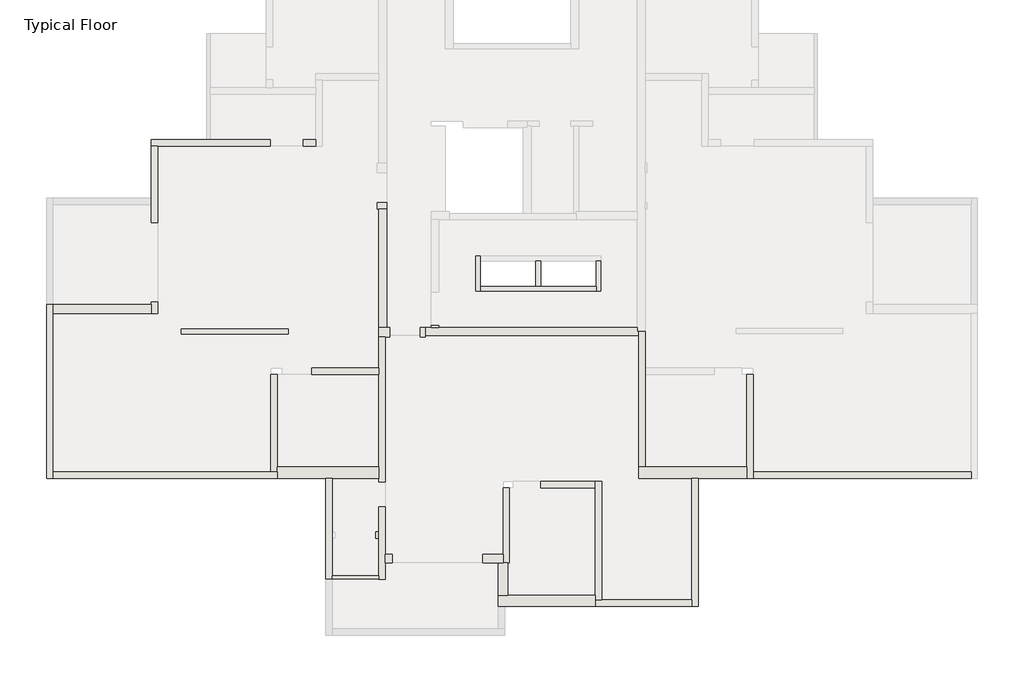
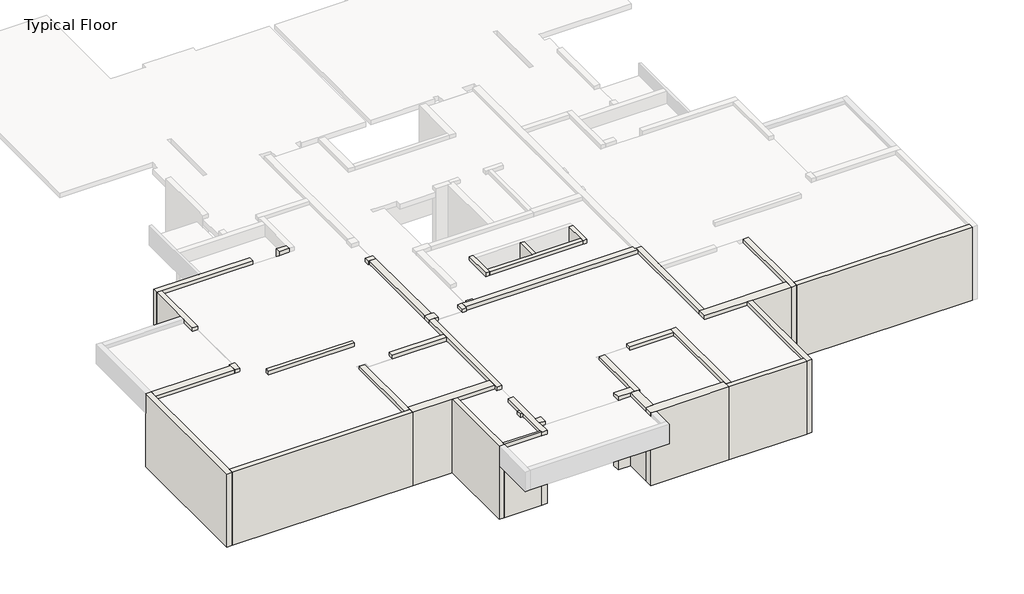
# One storey, part 1 of 4: 39 walls.
# Revit data of these elements (continued)
# Element 37 (IfcWall, "35") (continued)
#   SOFiSTiK_AMG_Adjusted = yes
#   Phase Created = New Construction
#   Base Constraint = Typical Floor
#   Top Constraint = Typical Floor
#   Materials on its faces: "Concrete, Cast-in-Place - B30"
# Element 38 (IfcWall, "35")
#   Comments = ""
#   Mark = "W72"
#   SOFiSTiK_AMG_Comments = ""
#   built-in parameter 1001111 = -300 cm
#   Top Offset = 0 cm
#   Base Offset = -300 cm
#   wall height = 300 cm
#   SOFiSTiK_AMG_Scheduled = yes
#   SOFiSTiK_AMG_Adjusted = yes
#   Phase Created = New Construction
#   Base Constraint = Typical Floor
#   Top Constraint = Typical Floor
#   Materials on its faces: "Concrete, Cast-in-Place - B30"
# Element 39 (IfcWall, "35")
#   Comments = ""
#   Mark = "W73"
#   SOFiSTiK_AMG_Comments = ""
#   built-in parameter 1001111 = -300 cm
#   Top Offset = 0 cm
#   Base Offset = -300 cm
#   wall height = 300 cm
#   SOFiSTiK_AMG_Scheduled = yes
#   SOFiSTiK_AMG_Adjusted = yes
#   Phase Created = New Construction
#   Base Constraint = Typical Floor
#   Top Constraint = Typical Floor
#   Materials on its faces: "Concrete, Cast-in-Place - B30"
# Materials
#   "Concrete, Cast-in-Place - B30": class "Concrete", colour RGB 192 192 192, transparency 0, Keynote = "01000", Description = "Cast-in-place concrete", Cost = 0
